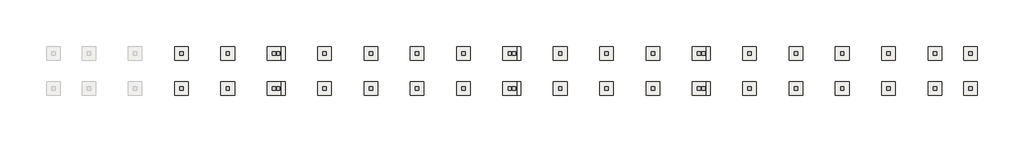
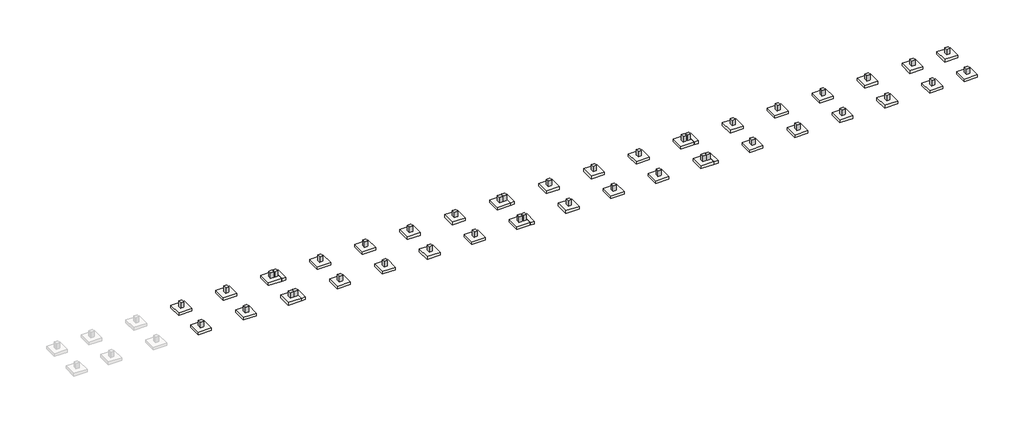
# Not in any storey, part 3 of 3: 42 columns, 42 slabs.
"""IFC4 building model written with IfcOpenShell, lengths in millimetres."""

import ifcopenshell
import ifcopenshell.guid

model = None  # the IFC model being written
_history = None  # IfcOwnerHistory: only IFC2X3 demands one
_inside = {}  # id of a spatial element -> (the spatial element, [elements in it])
_under = {}  # id of a project, library or spatial element -> (it, [spatial elements below it])
_declared = {}  # id of a project -> (the project, [libraries it declares])
_typed = {}  # id of a type object -> (the type object, [elements of that type])
_made_of = {}  # id of a material, layer set ... -> (it, [elements and type objects made of it])


def new_model(schema):
    """Start an empty IFC model of exactly this schema.

    Asked for "IFC4X3", IfcOpenShell would pick the latest addendum, in which some entities
    have other attributes; the version numbers below select the first issue.
    IFC2X3 requires an IfcOwnerHistory on every rooted entity: one is made here for all.
    """
    global model, _history
    if schema == "IFC4X3":
        model = ifcopenshell.file(schema_version=(4, 3, 0, 0))
    else:
        model = ifcopenshell.file(schema=schema)
    _inside.clear()
    _under.clear()
    _declared.clear()
    _typed.clear()
    _made_of.clear()
    _history = None
    if model.schema == "IFC2X3":
        org = make("IfcOrganization", Name="unknown")
        user = make(
            "IfcPersonAndOrganization",
            ThePerson=make("IfcPerson", FamilyName="unknown"),
            TheOrganization=org,
        )
        app = make(
            "IfcApplication",
            ApplicationDeveloper=org,
            Version="unknown",
            ApplicationFullName="unknown",
            ApplicationIdentifier="unknown",
        )
        _history = make(
            "IfcOwnerHistory",
            OwningUser=user,
            OwningApplication=app,
            ChangeAction="ADDED",
            CreationDate=0,
        )
    return model


def make(cls, **values):
    """One entity of the class cls with the attributes given. An attribute that is None is left unset."""
    return model.create_entity(
        cls, **{name: value for name, value in values.items() if value is not None}
    )


def rooted(cls, **values):
    """An entity with a GlobalId (a new one), such as an element, a storey or a relation."""
    return make(cls, GlobalId=ifcopenshell.guid.new(), OwnerHistory=_history, **values)


def si_unit(unit_type, name, prefix=None):
    """IfcSIUnit, for example si_unit("LENGTHUNIT", "METRE", prefix="MILLI")."""
    return make("IfcSIUnit", UnitType=unit_type, Prefix=prefix, Name=name)


def assignment(units):
    """IfcUnitAssignment: the units of a project."""
    return None if units is None else make("IfcUnitAssignment", Units=units)


def point(xyz):
    """IfcCartesianPoint."""
    return None if xyz is None else make("IfcCartesianPoint", Coordinates=xyz)


def direction(xyz):
    """IfcDirection."""
    return None if xyz is None else make("IfcDirection", DirectionRatios=xyz)


def frame(location, z_axis=None, x_axis=None):
    """IfcAxis2Placement3D, a coordinate frame: its origin and axes. An axis left out is left unset."""
    return make(
        "IfcAxis2Placement3D",
        Location=point(location),
        Axis=direction(z_axis),
        RefDirection=direction(x_axis),
    )


def origin():
    """The frame at (0, 0, 0) with its axes left unset."""
    return frame((0.0, 0.0, 0.0))


def place(relative_to, where):
    """IfcLocalPlacement: puts the frame where relative to a parent placement (None: the world)."""
    return make(
        "IfcLocalPlacement", PlacementRelTo=relative_to, RelativePlacement=where
    )


def context(
    kind, dimensions, precision=None, world=None, true_north=None, identifier=None
):
    """IfcGeometricRepresentationContext, for example the 3D "Model" context."""
    return make(
        "IfcGeometricRepresentationContext",
        ContextIdentifier=identifier,
        ContextType=kind,
        CoordinateSpaceDimension=dimensions,
        Precision=precision,
        WorldCoordinateSystem=world,
        TrueNorth=true_north,
    )


def project(units=None, contexts=None):
    """IfcProject with its units and contexts."""
    return rooted(
        "IfcProject",
        Name="project",
        RepresentationContexts=contexts,
        UnitsInContext=assignment(units),
    )


def spatial(cls, under=None, at=None, **own):
    """A site, building, storey or space (cls), placed at a placement, below another one or the project."""
    s = rooted(cls, ObjectPlacement=at, **own)
    if under is not None:
        _under.setdefault(under.id(), (under, []))[1].append(s)
    return s


def polyline(points):
    """IfcPolyline through the points."""
    return make("IfcPolyline", Points=[point(p) for p in points])


def outline(outer, holes=None, kind="AREA"):
    """IfcArbitraryClosedProfileDef: a profile drawn as a closed curve; with holes, ...WithVoids."""
    if holes is None:
        return make("IfcArbitraryClosedProfileDef", ProfileType=kind, OuterCurve=outer)
    return make(
        "IfcArbitraryProfileDefWithVoids",
        ProfileType=kind,
        OuterCurve=outer,
        InnerCurves=holes,
    )


def extrude(swept, where, along, depth):
    """IfcExtrudedAreaSolid: the profile swept, set in the frame where, extruded along a direction by depth."""
    return make(
        "IfcExtrudedAreaSolid",
        SweptArea=swept,
        Position=where,
        ExtrudedDirection=direction(along),
        Depth=depth,
    )


def shape(context_of_items, identifier, shape_type, items):
    """IfcShapeRepresentation: the items that make up one representation, for example the "Body"."""
    return make(
        "IfcShapeRepresentation",
        ContextOfItems=context_of_items,
        RepresentationIdentifier=identifier,
        RepresentationType=shape_type,
        Items=items,
    )


def source(mapping_origin, context_of_items, identifier, shape_type, items):
    """IfcRepresentationMap: a shape defined once, which mapped items show again and again."""
    return make(
        "IfcRepresentationMap",
        MappingOrigin=mapping_origin,
        MappedRepresentation=shape(context_of_items, identifier, shape_type, items),
    )


def transform(
    local_origin,
    x_axis=None,
    y_axis=None,
    z_axis=None,
    scale=None,
    scale2=None,
    scale3=None,
    uniform=True,
):
    """IfcCartesianTransformationOperator3D, or its non-uniform kind. x_axis, y_axis, z_axis: its Axis1, 2, 3."""
    if uniform:
        return make(
            "IfcCartesianTransformationOperator3D",
            Axis1=direction(x_axis),
            Axis2=direction(y_axis),
            LocalOrigin=point(local_origin),
            Scale=scale,
            Axis3=direction(z_axis),
        )
    return make(
        "IfcCartesianTransformationOperator3DnonUniform",
        Axis1=direction(x_axis),
        Axis2=direction(y_axis),
        LocalOrigin=point(local_origin),
        Scale=scale,
        Axis3=direction(z_axis),
        Scale2=scale2,
        Scale3=scale3,
    )


def mapped(mapping_source, mapping_target):
    """IfcMappedItem: shows the shape of a source again, moved by a transform."""
    return make(
        "IfcMappedItem", MappingSource=mapping_source, MappingTarget=mapping_target
    )


def made_of(thing, what):
    """Note that an element or type object is made of a material, layer set ...; save() writes the relation."""
    if what is not None:
        _made_of.setdefault(what.id(), (what, []))[1].append(thing)
    return thing


def element(
    cls,
    number,
    at=None,
    inside=None,
    cuts=None,
    type_object=None,
    material=None,
    context=None,
    identifier="Body",
    shape_type=None,
    held_by="IfcProductDefinitionShape",
    body=None,
    shapes=None,
    **own,
):
    """One element of the class cls, such as IfcWall. Its Tag is "e" and its number.

    at: its placement. inside: the storey or other place that contains it. cuts: it is an
    opening in that element (IfcRelVoidsElement). A single representation is given by context,
    identifier, shape_type and body (its items); several are given by shapes. held_by: the class
    of the entity that holds the representations. save() writes the other relations.
    """
    e = rooted(cls, Tag="e%d" % number, ObjectPlacement=at, **own)
    if body is not None:
        shapes = [shape(context, identifier, shape_type, body)]
    if shapes is not None:
        e.Representation = make(held_by, Representations=shapes)
    if inside is not None:
        _inside.setdefault(inside.id(), (inside, []))[1].append(e)
    if cuts is not None:
        rooted(
            "IfcRelVoidsElement", RelatingBuildingElement=cuts, RelatedOpeningElement=e
        )
    if type_object is not None:
        _typed.setdefault(type_object.id(), (type_object, []))[1].append(e)
    return made_of(e, material)


def aggregate(whole, parts):
    """IfcRelAggregates: a whole, such as a stair, and the parts it consists of."""
    return rooted("IfcRelAggregates", RelatingObject=whole, RelatedObjects=parts)


def save(model, path):
    """Write the relations noted so far, then the file.

    IfcRelAggregates (storeys below a building ...), IfcRelContainedInSpatialStructure (elements
    in a storey), IfcRelDefinesByType, IfcRelAssociatesMaterial and IfcRelDeclares: one each for
    every whole, place, type object, material and project.
    """
    for whole, parts in _under.values():
        aggregate(whole, parts)
    for where, things in _inside.values():
        rooted(
            "IfcRelContainedInSpatialStructure",
            RelatedElements=things,
            RelatingStructure=where,
        )
    for kind, things in _typed.values():
        rooted("IfcRelDefinesByType", RelatedObjects=things, RelatingType=kind)
    for what, things in _made_of.values():
        rooted("IfcRelAssociatesMaterial", RelatedObjects=things, RelatingMaterial=what)
    for by, libraries in _declared.values():
        rooted("IfcRelDeclares", RelatingContext=by, RelatedDefinitions=libraries)
    model.write(path)


def foundation_rectangular_non_pile_5fe39465(model_context):
    return source(origin(), model_context, "Body", "SweptSolid", [
        extrude(outline(polyline([(1200.0, 1200.0), (1200.0, -1200.0), (-1200.0, -1200.0), (-1200.0, 1200.0), (1200.0, 1200.0)])), frame((0.0, 0.0, -500.0), z_axis=(0.0, 0.0, 1.0), x_axis=(1.0, 0.0, 0.0)), (0.0, 0.0, 1.0), 500.0),
    ])


model = new_model("IFC4")

# Units and contexts
model_context = context("Model", 3, world=origin())
ifc_project = project(units=[si_unit("LENGTHUNIT", "METRE", prefix="MILLI")], contexts=[model_context])

# Site, building
site = spatial("IfcSite", under=ifc_project)
building = spatial("IfcBuilding", under=site)

# Columns
placement = place(None, origin())
element("IfcColumn", 1, ObjectType="RC_Column_Rectangular : H_SC_AR_S15_UG PED_W600xL600_Bit_Anchor", at=placement, inside=building, context=model_context, shape_type="SweptSolid", body=[
    extrude(outline(polyline([(18630.0, 549.5208589), (18630.0, -50.4791411), (18030.0, -50.4791411), (18030.0, 549.5208589), (18630.0, 549.5208589)])), frame((0.0, 0.0, -750.0381366), z_axis=(0.0, 0.0, 1.0), x_axis=(1.0, 0.0, 0.0)), (0.0, 0.0, 1.0), 1050.0),
])
element("IfcColumn", 2, ObjectType="RC_Column_Rectangular : H_SC_AR_S15_UG PED_W600xL600_Bit_Anchor", at=placement, inside=building, context=model_context, shape_type="SweptSolid", body=[
    extrude(outline(polyline([(26830.0, 549.5208589), (26830.0, -50.4791411), (26230.0, -50.4791411), (26230.0, 549.5208589), (26830.0, 549.5208589)])), frame((0.0, 0.0, -750.0381366), z_axis=(0.0, 0.0, 1.0), x_axis=(1.0, 0.0, 0.0)), (0.0, 0.0, 1.0), 1050.0),
])
element("IfcColumn", 3, ObjectType="RC_Column_Rectangular : H_SC_AR_S15_UG PED_W600xL600_Bit_Anchor", at=placement, inside=building, context=model_context, shape_type="SweptSolid", body=[
    extrude(outline(polyline([(35030.0, 549.5208589), (35030.0, -50.4791411), (34430.0, -50.4791411), (34430.0, 549.5208589), (35030.0, 549.5208589)])), frame((0.0, 0.0, -750.0381366), z_axis=(0.0, 0.0, 1.0), x_axis=(1.0, 0.0, 0.0)), (0.0, 0.0, 1.0), 1050.0),
])
element("IfcColumn", 4, ObjectType="RC_Column_Rectangular : H_SC_AR_S15_UG PED_W600xL600_Bit_Anchor", at=placement, inside=building, context=model_context, shape_type="SweptSolid", body=[
    extrude(outline(polyline([(35780.0, 549.5208589), (35780.0, -50.4791411), (35180.0, -50.4791411), (35180.0, 549.5208589), (35780.0, 549.5208589)])), frame((0.0, 0.0, -750.0381366), z_axis=(0.0, 0.0, 1.0), x_axis=(1.0, 0.0, 0.0)), (0.0, 0.0, 1.0), 1050.0),
])
element("IfcColumn", 5, ObjectType="RC_Column_Rectangular : H_SC_AR_S15_UG PED_W600xL600_Bit_Anchor", at=placement, inside=building, context=model_context, shape_type="SweptSolid", body=[
    extrude(outline(polyline([(43980.0, 549.5208589), (43980.0, -50.4791411), (43380.0, -50.4791411), (43380.0, 549.5208589), (43980.0, 549.5208589)])), frame((0.0, 0.0, -750.0381366), z_axis=(0.0, 0.0, 1.0), x_axis=(1.0, 0.0, 0.0)), (0.0, 0.0, 1.0), 1050.0),
])
element("IfcColumn", 6, ObjectType="RC_Column_Rectangular : H_SC_AR_S15_UG PED_W600xL600_Bit_Anchor", at=placement, inside=building, context=model_context, shape_type="SweptSolid", body=[
    extrude(outline(polyline([(52180.0, 549.5208589), (52180.0, -50.4791411), (51580.0, -50.4791411), (51580.0, 549.5208589), (52180.0, 549.5208589)])), frame((0.0, 0.0, -750.0381366), z_axis=(0.0, 0.0, 1.0), x_axis=(1.0, 0.0, 0.0)), (0.0, 0.0, 1.0), 1050.0),
])
element("IfcColumn", 7, ObjectType="RC_Column_Rectangular : H_SC_AR_S15_UG PED_W600xL600_Bit_Anchor", at=placement, inside=building, context=model_context, shape_type="SweptSolid", body=[
    extrude(outline(polyline([(60380.0, 549.5208589), (60380.0, -50.4791411), (59780.0, -50.4791411), (59780.0, 549.5208589), (60380.0, 549.5208589)])), frame((0.0, 0.0, -750.0381366), z_axis=(0.0, 0.0, 1.0), x_axis=(1.0, 0.0, 0.0)), (0.0, 0.0, 1.0), 1050.0),
])
element("IfcColumn", 8, ObjectType="RC_Column_Rectangular : H_SC_AR_S15_UG PED_W600xL600_Bit_Anchor", at=placement, inside=building, context=model_context, shape_type="SweptSolid", body=[
    extrude(outline(polyline([(68580.0, 549.5208589), (68580.0, -50.4791411), (67980.0, -50.4791411), (67980.0, 549.5208589), (68580.0, 549.5208589)])), frame((0.0, 0.0, -750.0381366), z_axis=(0.0, 0.0, 1.0), x_axis=(1.0, 0.0, 0.0)), (0.0, 0.0, 1.0), 1050.0),
])
element("IfcColumn", 9, ObjectType="RC_Column_Rectangular : H_SC_AR_S15_UG PED_W600xL600_Bit_Anchor", at=placement, inside=building, context=model_context, shape_type="SweptSolid", body=[
    extrude(outline(polyline([(76780.0, 549.5208589), (76780.0, -50.4791411), (76180.0, -50.4791411), (76180.0, 549.5208589), (76780.0, 549.5208589)])), frame((0.0, 0.0, -750.0381366), z_axis=(0.0, 0.0, 1.0), x_axis=(1.0, 0.0, 0.0)), (0.0, 0.0, 1.0), 1050.0),
])
element("IfcColumn", 10, ObjectType="RC_Column_Rectangular : H_SC_AR_S15_UG PED_W600xL600_Bit_Anchor", at=placement, inside=building, context=model_context, shape_type="SweptSolid", body=[
    extrude(outline(polyline([(77530.0, 549.5208589), (77530.0, -50.4791411), (76930.0, -50.4791411), (76930.0, 549.5208589), (77530.0, 549.5208589)])), frame((0.0, 0.0, -750.0381366), z_axis=(0.0, 0.0, 1.0), x_axis=(1.0, 0.0, 0.0)), (0.0, 0.0, 1.0), 1050.0),
])
element("IfcColumn", 11, ObjectType="RC_Column_Rectangular : H_SC_AR_S15_UG PED_W600xL600_Bit_Anchor", at=placement, inside=building, context=model_context, shape_type="SweptSolid", body=[
    extrude(outline(polyline([(85730.0, 549.5208589), (85730.0, -50.4791411), (85130.0, -50.4791411), (85130.0, 549.5208589), (85730.0, 549.5208589)])), frame((0.0, 0.0, -750.0381366), z_axis=(0.0, 0.0, 1.0), x_axis=(1.0, 0.0, 0.0)), (0.0, 0.0, 1.0), 1050.0),
])
element("IfcColumn", 12, ObjectType="RC_Column_Rectangular : H_SC_AR_S15_UG PED_W600xL600_Bit_Anchor", at=placement, inside=building, context=model_context, shape_type="SweptSolid", body=[
    extrude(outline(polyline([(93930.0, 549.5208589), (93930.0, -50.4791411), (93330.0, -50.4791411), (93330.0, 549.5208589), (93930.0, 549.5208589)])), frame((0.0, 0.0, -750.0381366), z_axis=(0.0, 0.0, 1.0), x_axis=(1.0, 0.0, 0.0)), (0.0, 0.0, 1.0), 1050.0),
])
element("IfcColumn", 13, ObjectType="RC_Column_Rectangular : H_SC_AR_S15_UG PED_W600xL600_Bit_Anchor", at=placement, inside=building, context=model_context, shape_type="SweptSolid", body=[
    extrude(outline(polyline([(102130.0, 549.5208589), (102130.0, -50.4791411), (101530.0, -50.4791411), (101530.0, 549.5208589), (102130.0, 549.5208589)])), frame((0.0, 0.0, -750.0381366), z_axis=(0.0, 0.0, 1.0), x_axis=(1.0, 0.0, 0.0)), (0.0, 0.0, 1.0), 1050.0),
])
element("IfcColumn", 14, ObjectType="RC_Column_Rectangular : H_SC_AR_S15_UG PED_W600xL600_Bit_Anchor", at=placement, inside=building, context=model_context, shape_type="SweptSolid", body=[
    extrude(outline(polyline([(110330.0, 549.5208589), (110330.0, -50.4791411), (109730.0, -50.4791411), (109730.0, 549.5208589), (110330.0, 549.5208589)])), frame((0.0, 0.0, -750.0381366), z_axis=(0.0, 0.0, 1.0), x_axis=(1.0, 0.0, 0.0)), (0.0, 0.0, 1.0), 1050.0),
])
element("IfcColumn", 15, ObjectType="RC_Column_Rectangular : H_SC_AR_S15_UG PED_W600xL600_Bit_Anchor", at=placement, inside=building, context=model_context, shape_type="SweptSolid", body=[
    extrude(outline(polyline([(111080.0, 549.5208589), (111080.0, -50.4791411), (110480.0, -50.4791411), (110480.0, 549.5208589), (111080.0, 549.5208589)])), frame((0.0, 0.0, -750.0381366), z_axis=(0.0, 0.0, 1.0), x_axis=(1.0, 0.0, 0.0)), (0.0, 0.0, 1.0), 1050.0),
])
element("IfcColumn", 16, ObjectType="RC_Column_Rectangular : H_SC_AR_S15_UG PED_W600xL600_Bit_Anchor", at=placement, inside=building, context=model_context, shape_type="SweptSolid", body=[
    extrude(outline(polyline([(119280.0, 549.5208589), (119280.0, -50.4791411), (118680.0, -50.4791411), (118680.0, 549.5208589), (119280.0, 549.5208589)])), frame((0.0, 0.0, -750.0381366), z_axis=(0.0, 0.0, 1.0), x_axis=(1.0, 0.0, 0.0)), (0.0, 0.0, 1.0), 1050.0),
])
element("IfcColumn", 17, ObjectType="RC_Column_Rectangular : H_SC_AR_S15_UG PED_W600xL600_Bit_Anchor", at=placement, inside=building, context=model_context, shape_type="SweptSolid", body=[
    extrude(outline(polyline([(127480.0, 549.5208589), (127480.0, -50.4791411), (126880.0, -50.4791411), (126880.0, 549.5208589), (127480.0, 549.5208589)])), frame((0.0, 0.0, -750.0381366), z_axis=(0.0, 0.0, 1.0), x_axis=(1.0, 0.0, 0.0)), (0.0, 0.0, 1.0), 1050.0),
])
element("IfcColumn", 18, ObjectType="RC_Column_Rectangular : H_SC_AR_S15_UG PED_W600xL600_Bit_Anchor", at=placement, inside=building, context=model_context, shape_type="SweptSolid", body=[
    extrude(outline(polyline([(135680.0, 549.5208589), (135680.0, -50.4791411), (135080.0, -50.4791411), (135080.0, 549.5208589), (135680.0, 549.5208589)])), frame((0.0, 0.0, -750.0381366), z_axis=(0.0, 0.0, 1.0), x_axis=(1.0, 0.0, 0.0)), (0.0, 0.0, 1.0), 1050.0),
])
element("IfcColumn", 19, ObjectType="RC_Column_Rectangular : H_SC_AR_S15_UG PED_W600xL600_Bit_Anchor", at=placement, inside=building, context=model_context, shape_type="SweptSolid", body=[
    extrude(outline(polyline([(143880.0, 549.5208589), (143880.0, -50.4791411), (143280.0, -50.4791411), (143280.0, 549.5208589), (143880.0, 549.5208589)])), frame((0.0, 0.0, -750.0381366), z_axis=(0.0, 0.0, 1.0), x_axis=(1.0, 0.0, 0.0)), (0.0, 0.0, 1.0), 1050.0),
])
element("IfcColumn", 20, ObjectType="RC_Column_Rectangular : H_SC_AR_S15_UG PED_W600xL600_Bit_Anchor", at=placement, inside=building, context=model_context, shape_type="SweptSolid", body=[
    extrude(outline(polyline([(152080.0, 549.5208589), (152080.0, -50.4791411), (151480.0, -50.4791411), (151480.0, 549.5208589), (152080.0, 549.5208589)])), frame((0.0, 0.0, -750.0381366), z_axis=(0.0, 0.0, 1.0), x_axis=(1.0, 0.0, 0.0)), (0.0, 0.0, 1.0), 1050.0),
])
element("IfcColumn", 21, ObjectType="RC_Column_Rectangular : H_SC_AR_S15_UG PED_W600xL600_Bit_Anchor", at=placement, inside=building, context=model_context, shape_type="SweptSolid", body=[
    extrude(outline(polyline([(158430.0, 549.5208589), (158430.0, -50.4791411), (157830.0, -50.4791411), (157830.0, 549.5208589), (158430.0, 549.5208589)])), frame((0.0, 0.0, -750.0381366), z_axis=(0.0, 0.0, 1.0), x_axis=(1.0, 0.0, 0.0)), (0.0, 0.0, 1.0), 1050.0),
])
element("IfcColumn", 22, ObjectType="RC_Column_Rectangular : H_SC_AR_S15_UG PED_W600xL600_Bit_Anchor", at=placement, inside=building, context=model_context, shape_type="SweptSolid", body=[
    extrude(outline(polyline([(18630.0, 6799.5208589), (18630.0, 6199.5208589), (18030.0, 6199.5208589), (18030.0, 6799.5208589), (18630.0, 6799.5208589)])), frame((0.0, 0.0, -750.0381366), z_axis=(0.0, 0.0, 1.0), x_axis=(1.0, 0.0, 0.0)), (0.0, 0.0, 1.0), 1050.0),
])
element("IfcColumn", 23, ObjectType="RC_Column_Rectangular : H_SC_AR_S15_UG PED_W600xL600_Bit_Anchor", at=placement, inside=building, context=model_context, shape_type="SweptSolid", body=[
    extrude(outline(polyline([(26830.0, 6799.5208589), (26830.0, 6199.5208589), (26230.0, 6199.5208589), (26230.0, 6799.5208589), (26830.0, 6799.5208589)])), frame((0.0, 0.0, -750.0381366), z_axis=(0.0, 0.0, 1.0), x_axis=(1.0, 0.0, 0.0)), (0.0, 0.0, 1.0), 1050.0),
])
element("IfcColumn", 24, ObjectType="RC_Column_Rectangular : H_SC_AR_S15_UG PED_W600xL600_Bit_Anchor", at=placement, inside=building, context=model_context, shape_type="SweptSolid", body=[
    extrude(outline(polyline([(35030.0, 6799.5208589), (35030.0, 6199.5208589), (34430.0, 6199.5208589), (34430.0, 6799.5208589), (35030.0, 6799.5208589)])), frame((0.0, 0.0, -750.0381366), z_axis=(0.0, 0.0, 1.0), x_axis=(1.0, 0.0, 0.0)), (0.0, 0.0, 1.0), 1050.0),
])
element("IfcColumn", 25, ObjectType="RC_Column_Rectangular : H_SC_AR_S15_UG PED_W600xL600_Bit_Anchor", at=placement, inside=building, context=model_context, shape_type="SweptSolid", body=[
    extrude(outline(polyline([(35780.0, 6799.5208589), (35780.0, 6199.5208589), (35180.0, 6199.5208589), (35180.0, 6799.5208589), (35780.0, 6799.5208589)])), frame((0.0, 0.0, -750.0381366), z_axis=(0.0, 0.0, 1.0), x_axis=(1.0, 0.0, 0.0)), (0.0, 0.0, 1.0), 1050.0),
])
element("IfcColumn", 26, ObjectType="RC_Column_Rectangular : H_SC_AR_S15_UG PED_W600xL600_Bit_Anchor", at=placement, inside=building, context=model_context, shape_type="SweptSolid", body=[
    extrude(outline(polyline([(43980.0, 6799.5208589), (43980.0, 6199.5208589), (43380.0, 6199.5208589), (43380.0, 6799.5208589), (43980.0, 6799.5208589)])), frame((0.0, 0.0, -750.0381366), z_axis=(0.0, 0.0, 1.0), x_axis=(1.0, 0.0, 0.0)), (0.0, 0.0, 1.0), 1050.0),
])
element("IfcColumn", 27, ObjectType="RC_Column_Rectangular : H_SC_AR_S15_UG PED_W600xL600_Bit_Anchor", at=placement, inside=building, context=model_context, shape_type="SweptSolid", body=[
    extrude(outline(polyline([(52180.0, 6799.5208589), (52180.0, 6199.5208589), (51580.0, 6199.5208589), (51580.0, 6799.5208589), (52180.0, 6799.5208589)])), frame((0.0, 0.0, -750.0381366), z_axis=(0.0, 0.0, 1.0), x_axis=(1.0, 0.0, 0.0)), (0.0, 0.0, 1.0), 1050.0),
])
element("IfcColumn", 28, ObjectType="RC_Column_Rectangular : H_SC_AR_S15_UG PED_W600xL600_Bit_Anchor", at=placement, inside=building, context=model_context, shape_type="SweptSolid", body=[
    extrude(outline(polyline([(60380.0, 6799.5208589), (60380.0, 6199.5208589), (59780.0, 6199.5208589), (59780.0, 6799.5208589), (60380.0, 6799.5208589)])), frame((0.0, 0.0, -750.0381366), z_axis=(0.0, 0.0, 1.0), x_axis=(1.0, 0.0, 0.0)), (0.0, 0.0, 1.0), 1050.0),
])
element("IfcColumn", 29, ObjectType="RC_Column_Rectangular : H_SC_AR_S15_UG PED_W600xL600_Bit_Anchor", at=placement, inside=building, context=model_context, shape_type="SweptSolid", body=[
    extrude(outline(polyline([(68580.0, 6799.5208589), (68580.0, 6199.5208589), (67980.0, 6199.5208589), (67980.0, 6799.5208589), (68580.0, 6799.5208589)])), frame((0.0, 0.0, -750.0381366), z_axis=(0.0, 0.0, 1.0), x_axis=(1.0, 0.0, 0.0)), (0.0, 0.0, 1.0), 1050.0),
])
element("IfcColumn", 30, ObjectType="RC_Column_Rectangular : H_SC_AR_S15_UG PED_W600xL600_Bit_Anchor", at=placement, inside=building, context=model_context, shape_type="SweptSolid", body=[
    extrude(outline(polyline([(76780.0, 6799.5208589), (76780.0, 6199.5208589), (76180.0, 6199.5208589), (76180.0, 6799.5208589), (76780.0, 6799.5208589)])), frame((0.0, 0.0, -750.0381366), z_axis=(0.0, 0.0, 1.0), x_axis=(1.0, 0.0, 0.0)), (0.0, 0.0, 1.0), 1050.0),
])
element("IfcColumn", 31, ObjectType="RC_Column_Rectangular : H_SC_AR_S15_UG PED_W600xL600_Bit_Anchor", at=placement, inside=building, context=model_context, shape_type="SweptSolid", body=[
    extrude(outline(polyline([(77530.0, 6799.5208589), (77530.0, 6199.5208589), (76930.0, 6199.5208589), (76930.0, 6799.5208589), (77530.0, 6799.5208589)])), frame((0.0, 0.0, -750.0381366), z_axis=(0.0, 0.0, 1.0), x_axis=(1.0, 0.0, 0.0)), (0.0, 0.0, 1.0), 1050.0),
])
element("IfcColumn", 32, ObjectType="RC_Column_Rectangular : H_SC_AR_S15_UG PED_W600xL600_Bit_Anchor", at=placement, inside=building, context=model_context, shape_type="SweptSolid", body=[
    extrude(outline(polyline([(85730.0, 6799.5208589), (85730.0, 6199.5208589), (85130.0, 6199.5208589), (85130.0, 6799.5208589), (85730.0, 6799.5208589)])), frame((0.0, 0.0, -750.0381366), z_axis=(0.0, 0.0, 1.0), x_axis=(1.0, 0.0, 0.0)), (0.0, 0.0, 1.0), 1050.0),
])
element("IfcColumn", 33, ObjectType="RC_Column_Rectangular : H_SC_AR_S15_UG PED_W600xL600_Bit_Anchor", at=placement, inside=building, context=model_context, shape_type="SweptSolid", body=[
    extrude(outline(polyline([(93930.0, 6799.5208589), (93930.0, 6199.5208589), (93330.0, 6199.5208589), (93330.0, 6799.5208589), (93930.0, 6799.5208589)])), frame((0.0, 0.0, -750.0381366), z_axis=(0.0, 0.0, 1.0), x_axis=(1.0, 0.0, 0.0)), (0.0, 0.0, 1.0), 1050.0),
])
element("IfcColumn", 34, ObjectType="RC_Column_Rectangular : H_SC_AR_S15_UG PED_W600xL600_Bit_Anchor", at=placement, inside=building, context=model_context, shape_type="SweptSolid", body=[
    extrude(outline(polyline([(102130.0, 6799.5208589), (102130.0, 6199.5208589), (101530.0, 6199.5208589), (101530.0, 6799.5208589), (102130.0, 6799.5208589)])), frame((0.0, 0.0, -750.0381366), z_axis=(0.0, 0.0, 1.0), x_axis=(1.0, 0.0, 0.0)), (0.0, 0.0, 1.0), 1050.0),
])
element("IfcColumn", 35, ObjectType="RC_Column_Rectangular : H_SC_AR_S15_UG PED_W600xL600_Bit_Anchor", at=placement, inside=building, context=model_context, shape_type="SweptSolid", body=[
    extrude(outline(polyline([(110330.0, 6799.5208589), (110330.0, 6199.5208589), (109730.0, 6199.5208589), (109730.0, 6799.5208589), (110330.0, 6799.5208589)])), frame((0.0, 0.0, -750.0381366), z_axis=(0.0, 0.0, 1.0), x_axis=(1.0, 0.0, 0.0)), (0.0, 0.0, 1.0), 1050.0),
])
element("IfcColumn", 36, ObjectType="RC_Column_Rectangular : H_SC_AR_S15_UG PED_W600xL600_Bit_Anchor", at=placement, inside=building, context=model_context, shape_type="SweptSolid", body=[
    extrude(outline(polyline([(111080.0, 6799.5208589), (111080.0, 6199.5208589), (110480.0, 6199.5208589), (110480.0, 6799.5208589), (111080.0, 6799.5208589)])), frame((0.0, 0.0, -750.0381366), z_axis=(0.0, 0.0, 1.0), x_axis=(1.0, 0.0, 0.0)), (0.0, 0.0, 1.0), 1050.0),
])
element("IfcColumn", 37, ObjectType="RC_Column_Rectangular : H_SC_AR_S15_UG PED_W600xL600_Bit_Anchor", at=placement, inside=building, context=model_context, shape_type="SweptSolid", body=[
    extrude(outline(polyline([(119280.0, 6799.5208589), (119280.0, 6199.5208589), (118680.0, 6199.5208589), (118680.0, 6799.5208589), (119280.0, 6799.5208589)])), frame((0.0, 0.0, -750.0381366), z_axis=(0.0, 0.0, 1.0), x_axis=(1.0, 0.0, 0.0)), (0.0, 0.0, 1.0), 1050.0),
])
element("IfcColumn", 38, ObjectType="RC_Column_Rectangular : H_SC_AR_S15_UG PED_W600xL600_Bit_Anchor", at=placement, inside=building, context=model_context, shape_type="SweptSolid", body=[
    extrude(outline(polyline([(127480.0, 6799.5208589), (127480.0, 6199.5208589), (126880.0, 6199.5208589), (126880.0, 6799.5208589), (127480.0, 6799.5208589)])), frame((0.0, 0.0, -750.0381366), z_axis=(0.0, 0.0, 1.0), x_axis=(1.0, 0.0, 0.0)), (0.0, 0.0, 1.0), 1050.0),
])
element("IfcColumn", 39, ObjectType="RC_Column_Rectangular : H_SC_AR_S15_UG PED_W600xL600_Bit_Anchor", at=placement, inside=building, context=model_context, shape_type="SweptSolid", body=[
    extrude(outline(polyline([(135680.0, 6799.5208589), (135680.0, 6199.5208589), (135080.0, 6199.5208589), (135080.0, 6799.5208589), (135680.0, 6799.5208589)])), frame((0.0, 0.0, -750.0381366), z_axis=(0.0, 0.0, 1.0), x_axis=(1.0, 0.0, 0.0)), (0.0, 0.0, 1.0), 1050.0),
])
element("IfcColumn", 40, ObjectType="RC_Column_Rectangular : H_SC_AR_S15_UG PED_W600xL600_Bit_Anchor", at=placement, inside=building, context=model_context, shape_type="SweptSolid", body=[
    extrude(outline(polyline([(143880.0, 6799.5208589), (143880.0, 6199.5208589), (143280.0, 6199.5208589), (143280.0, 6799.5208589), (143880.0, 6799.5208589)])), frame((0.0, 0.0, -750.0381366), z_axis=(0.0, 0.0, 1.0), x_axis=(1.0, 0.0, 0.0)), (0.0, 0.0, 1.0), 1050.0),
])
element("IfcColumn", 41, ObjectType="RC_Column_Rectangular : H_SC_AR_S15_UG PED_W600xL600_Bit_Anchor", at=placement, inside=building, context=model_context, shape_type="SweptSolid", body=[
    extrude(outline(polyline([(152080.0, 6799.5208589), (152080.0, 6199.5208589), (151480.0, 6199.5208589), (151480.0, 6799.5208589), (152080.0, 6799.5208589)])), frame((0.0, 0.0, -750.0381366), z_axis=(0.0, 0.0, 1.0), x_axis=(1.0, 0.0, 0.0)), (0.0, 0.0, 1.0), 1050.0),
])
element("IfcColumn", 42, ObjectType="RC_Column_Rectangular : H_SC_AR_S15_UG PED_W600xL600_Bit_Anchor", at=placement, inside=building, context=model_context, shape_type="SweptSolid", body=[
    extrude(outline(polyline([(158430.0, 6799.5208589), (158430.0, 6199.5208589), (157830.0, 6199.5208589), (157830.0, 6799.5208589), (158430.0, 6799.5208589)])), frame((0.0, 0.0, -750.0381366), z_axis=(0.0, 0.0, 1.0), x_axis=(1.0, 0.0, 0.0)), (0.0, 0.0, 1.0), 1050.0),
])

# Slabs
element("IfcSlab", 43, ObjectType="Foundation Rectangular (Non-Pile) : H_SF_AR_S18_W2400xL2400xT500_Bitumen", at=placement, inside=building, context=model_context, shape_type="SweptSolid", body=[
    extrude(outline(polyline([(35930.0, 1449.5208589), (35930.0, -950.4791411), (33530.0, -950.4791411), (33530.0, 1449.5208589), (35930.0, 1449.5208589)])), frame((0.0, 0.0, -1250.0381366), z_axis=(0.0, 0.0, 1.0), x_axis=(1.0, 0.0, 0.0)), (0.0, 0.0, 1.0), 500.0),
])
element("IfcSlab", 44, ObjectType="Foundation Rectangular (Non-Pile) : H_SF_AR_S18_W2400xL2400xT500_Bitumen", at=placement, inside=building, context=model_context, shape_type="SweptSolid", body=[
    extrude(outline(polyline([(36680.0, 1449.5208589), (36680.0, -950.4791411), (35930.0, -950.4791411), (35930.0, 1449.5208589), (36680.0, 1449.5208589)])), frame((0.0, 0.0, -1250.0381366), z_axis=(0.0, 0.0, 1.0), x_axis=(1.0, 0.0, 0.0)), (0.0, 0.0, 1.0), 500.0),
])
element("IfcSlab", 45, ObjectType="Foundation Rectangular (Non-Pile) : H_SF_AR_S18_W2400xL2400xT500_Bitumen", at=placement, inside=building, context=model_context, shape_type="SweptSolid", body=[
    extrude(outline(polyline([(77680.0, 1449.5208589), (77680.0, -950.4791411), (75280.0, -950.4791411), (75280.0, 1449.5208589), (77680.0, 1449.5208589)])), frame((0.0, 0.0, -1250.0381366), z_axis=(0.0, 0.0, 1.0), x_axis=(1.0, 0.0, 0.0)), (0.0, 0.0, 1.0), 500.0),
])
element("IfcSlab", 46, ObjectType="Foundation Rectangular (Non-Pile) : H_SF_AR_S18_W2400xL2400xT500_Bitumen", at=placement, inside=building, context=model_context, shape_type="SweptSolid", body=[
    extrude(outline(polyline([(78430.0, 1449.5208589), (78430.0, -950.4791411), (77680.0, -950.4791411), (77680.0, 1449.5208589), (78430.0, 1449.5208589)])), frame((0.0, 0.0, -1250.0381366), z_axis=(0.0, 0.0, 1.0), x_axis=(1.0, 0.0, 0.0)), (0.0, 0.0, 1.0), 500.0),
])
element("IfcSlab", 47, ObjectType="Foundation Rectangular (Non-Pile) : H_SF_AR_S18_W2400xL2400xT500_Bitumen", at=placement, inside=building, context=model_context, shape_type="SweptSolid", body=[
    extrude(outline(polyline([(111230.0, 1449.5208589), (111230.0, -950.4791411), (108830.0, -950.4791411), (108830.0, 1449.5208589), (111230.0, 1449.5208589)])), frame((0.0, 0.0, -1250.0381366), z_axis=(0.0, 0.0, 1.0), x_axis=(1.0, 0.0, 0.0)), (0.0, 0.0, 1.0), 500.0),
])
element("IfcSlab", 48, ObjectType="Foundation Rectangular (Non-Pile) : H_SF_AR_S18_W2400xL2400xT500_Bitumen", at=placement, inside=building, context=model_context, shape_type="SweptSolid", body=[
    extrude(outline(polyline([(111980.0, 1449.5208589), (111980.0, -950.4791411), (111230.0, -950.4791411), (111230.0, 1449.5208589), (111980.0, 1449.5208589)])), frame((0.0, 0.0, -1250.0381366), z_axis=(0.0, 0.0, 1.0), x_axis=(1.0, 0.0, 0.0)), (0.0, 0.0, 1.0), 500.0),
])
element("IfcSlab", 49, ObjectType="Foundation Rectangular (Non-Pile) : H_SF_AR_S18_W2400xL2400xT500_Bitumen", at=placement, inside=building, context=model_context, shape_type="SweptSolid", body=[
    extrude(outline(polyline([(35930.0, 7699.5208589), (35930.0, 5299.5208589), (33530.0, 5299.5208589), (33530.0, 7699.5208589), (35930.0, 7699.5208589)])), frame((0.0, 0.0, -1250.0381366), z_axis=(0.0, 0.0, 1.0), x_axis=(1.0, 0.0, 0.0)), (0.0, 0.0, 1.0), 500.0),
])
element("IfcSlab", 50, ObjectType="Foundation Rectangular (Non-Pile) : H_SF_AR_S18_W2400xL2400xT500_Bitumen", at=placement, inside=building, context=model_context, shape_type="SweptSolid", body=[
    extrude(outline(polyline([(36680.0, 7699.5208589), (36680.0, 5299.5208589), (35930.0, 5299.5208589), (35930.0, 7699.5208589), (36680.0, 7699.5208589)])), frame((0.0, 0.0, -1250.0381366), z_axis=(0.0, 0.0, 1.0), x_axis=(1.0, 0.0, 0.0)), (0.0, 0.0, 1.0), 500.0),
])
element("IfcSlab", 51, ObjectType="Foundation Rectangular (Non-Pile) : H_SF_AR_S18_W2400xL2400xT500_Bitumen", at=placement, inside=building, context=model_context, shape_type="SweptSolid", body=[
    extrude(outline(polyline([(77680.0, 7699.5208589), (77680.0, 5299.5208589), (75280.0, 5299.5208589), (75280.0, 7699.5208589), (77680.0, 7699.5208589)])), frame((0.0, 0.0, -1250.0381366), z_axis=(0.0, 0.0, 1.0), x_axis=(1.0, 0.0, 0.0)), (0.0, 0.0, 1.0), 500.0),
])
element("IfcSlab", 52, ObjectType="Foundation Rectangular (Non-Pile) : H_SF_AR_S18_W2400xL2400xT500_Bitumen", at=placement, inside=building, context=model_context, shape_type="SweptSolid", body=[
    extrude(outline(polyline([(78430.0, 7699.5208589), (78430.0, 5299.5208589), (77680.0, 5299.5208589), (77680.0, 7699.5208589), (78430.0, 7699.5208589)])), frame((0.0, 0.0, -1250.0381366), z_axis=(0.0, 0.0, 1.0), x_axis=(1.0, 0.0, 0.0)), (0.0, 0.0, 1.0), 500.0),
])
element("IfcSlab", 53, ObjectType="Foundation Rectangular (Non-Pile) : H_SF_AR_S18_W2400xL2400xT500_Bitumen", at=placement, inside=building, context=model_context, shape_type="SweptSolid", body=[
    extrude(outline(polyline([(111230.0, 7699.5208589), (111230.0, 5299.5208589), (108830.0, 5299.5208589), (108830.0, 7699.5208589), (111230.0, 7699.5208589)])), frame((0.0, 0.0, -1250.0381366), z_axis=(0.0, 0.0, 1.0), x_axis=(1.0, 0.0, 0.0)), (0.0, 0.0, 1.0), 500.0),
])
element("IfcSlab", 54, ObjectType="Foundation Rectangular (Non-Pile) : H_SF_AR_S18_W2400xL2400xT500_Bitumen", at=placement, inside=building, context=model_context, shape_type="SweptSolid", body=[
    extrude(outline(polyline([(111980.0, 7699.5208589), (111980.0, 5299.5208589), (111230.0, 5299.5208589), (111230.0, 7699.5208589), (111980.0, 7699.5208589)])), frame((0.0, 0.0, -1250.0381366), z_axis=(0.0, 0.0, 1.0), x_axis=(1.0, 0.0, 0.0)), (0.0, 0.0, 1.0), 500.0),
])
foundation_rectangular_non_pile_shape = foundation_rectangular_non_pile_5fe39465(model_context)
element("IfcSlab", 55, ObjectType="Foundation Rectangular (Non-Pile) : H_SF_AR_S18_W2400xL2400xT500_Bitumen", at=placement, inside=building, context=model_context, shape_type="MappedRepresentation", body=[
    mapped(foundation_rectangular_non_pile_shape, transform((18330.0, 249.5208589, -750.0381366), x_axis=(1.0, 0.0, 0.0), y_axis=(0.0, 1.0, 0.0), z_axis=(0.0, 0.0, 1.0))),
])
element("IfcSlab", 56, ObjectType="Foundation Rectangular (Non-Pile) : H_SF_AR_S18_W2400xL2400xT500_Bitumen", at=placement, inside=building, context=model_context, shape_type="MappedRepresentation", body=[
    mapped(foundation_rectangular_non_pile_shape, transform((26530.0, 249.5208589, -750.0381366), x_axis=(1.0, 0.0, 0.0), y_axis=(0.0, 1.0, 0.0), z_axis=(0.0, 0.0, 1.0))),
])
element("IfcSlab", 57, ObjectType="Foundation Rectangular (Non-Pile) : H_SF_AR_S18_W2400xL2400xT500_Bitumen", at=placement, inside=building, context=model_context, shape_type="MappedRepresentation", body=[
    mapped(foundation_rectangular_non_pile_shape, transform((43680.0, 249.5208589, -750.0381366), x_axis=(1.0, 0.0, 0.0), y_axis=(0.0, 1.0, 0.0), z_axis=(0.0, 0.0, 1.0))),
])
element("IfcSlab", 58, ObjectType="Foundation Rectangular (Non-Pile) : H_SF_AR_S18_W2400xL2400xT500_Bitumen", at=placement, inside=building, context=model_context, shape_type="MappedRepresentation", body=[
    mapped(foundation_rectangular_non_pile_shape, transform((51880.0, 249.5208589, -750.0381366), x_axis=(1.0, 0.0, 0.0), y_axis=(0.0, 1.0, 0.0), z_axis=(0.0, 0.0, 1.0))),
])
element("IfcSlab", 59, ObjectType="Foundation Rectangular (Non-Pile) : H_SF_AR_S18_W2400xL2400xT500_Bitumen", at=placement, inside=building, context=model_context, shape_type="MappedRepresentation", body=[
    mapped(foundation_rectangular_non_pile_shape, transform((60080.0, 249.5208589, -750.0381366), x_axis=(1.0, 0.0, 0.0), y_axis=(0.0, 1.0, 0.0), z_axis=(0.0, 0.0, 1.0))),
])
element("IfcSlab", 60, ObjectType="Foundation Rectangular (Non-Pile) : H_SF_AR_S18_W2400xL2400xT500_Bitumen", at=placement, inside=building, context=model_context, shape_type="MappedRepresentation", body=[
    mapped(foundation_rectangular_non_pile_shape, transform((68280.0, 249.5208589, -750.0381366), x_axis=(1.0, 0.0, 0.0), y_axis=(0.0, 1.0, 0.0), z_axis=(0.0, 0.0, 1.0))),
])
element("IfcSlab", 61, ObjectType="Foundation Rectangular (Non-Pile) : H_SF_AR_S18_W2400xL2400xT500_Bitumen", at=placement, inside=building, context=model_context, shape_type="MappedRepresentation", body=[
    mapped(foundation_rectangular_non_pile_shape, transform((85430.0, 249.5208589, -750.0381366), x_axis=(1.0, 0.0, 0.0), y_axis=(0.0, 1.0, 0.0), z_axis=(0.0, 0.0, 1.0))),
])
element("IfcSlab", 62, ObjectType="Foundation Rectangular (Non-Pile) : H_SF_AR_S18_W2400xL2400xT500_Bitumen", at=placement, inside=building, context=model_context, shape_type="MappedRepresentation", body=[
    mapped(foundation_rectangular_non_pile_shape, transform((93630.0, 249.5208589, -750.0381366), x_axis=(1.0, 0.0, 0.0), y_axis=(0.0, 1.0, 0.0), z_axis=(0.0, 0.0, 1.0))),
])
element("IfcSlab", 63, ObjectType="Foundation Rectangular (Non-Pile) : H_SF_AR_S18_W2400xL2400xT500_Bitumen", at=placement, inside=building, context=model_context, shape_type="MappedRepresentation", body=[
    mapped(foundation_rectangular_non_pile_shape, transform((101830.0, 249.5208589, -750.0381366), x_axis=(1.0, 0.0, 0.0), y_axis=(0.0, 1.0, 0.0), z_axis=(0.0, 0.0, 1.0))),
])
element("IfcSlab", 64, ObjectType="Foundation Rectangular (Non-Pile) : H_SF_AR_S18_W2400xL2400xT500_Bitumen", at=placement, inside=building, context=model_context, shape_type="MappedRepresentation", body=[
    mapped(foundation_rectangular_non_pile_shape, transform((118980.0, 249.5208589, -750.0381366), x_axis=(1.0, 0.0, 0.0), y_axis=(0.0, 1.0, 0.0), z_axis=(0.0, 0.0, 1.0))),
])
element("IfcSlab", 65, ObjectType="Foundation Rectangular (Non-Pile) : H_SF_AR_S18_W2400xL2400xT500_Bitumen", at=placement, inside=building, context=model_context, shape_type="MappedRepresentation", body=[
    mapped(foundation_rectangular_non_pile_shape, transform((127180.0, 249.5208589, -750.0381366), x_axis=(1.0, 0.0, 0.0), y_axis=(0.0, 1.0, 0.0), z_axis=(0.0, 0.0, 1.0))),
])
element("IfcSlab", 66, ObjectType="Foundation Rectangular (Non-Pile) : H_SF_AR_S18_W2400xL2400xT500_Bitumen", at=placement, inside=building, context=model_context, shape_type="MappedRepresentation", body=[
    mapped(foundation_rectangular_non_pile_shape, transform((135380.0, 249.5208589, -750.0381366), x_axis=(1.0, 0.0, 0.0), y_axis=(0.0, 1.0, 0.0), z_axis=(0.0, 0.0, 1.0))),
])
element("IfcSlab", 67, ObjectType="Foundation Rectangular (Non-Pile) : H_SF_AR_S18_W2400xL2400xT500_Bitumen", at=placement, inside=building, context=model_context, shape_type="MappedRepresentation", body=[
    mapped(foundation_rectangular_non_pile_shape, transform((143580.0, 249.5208589, -750.0381366), x_axis=(1.0, 0.0, 0.0), y_axis=(0.0, 1.0, 0.0), z_axis=(0.0, 0.0, 1.0))),
])
element("IfcSlab", 68, ObjectType="Foundation Rectangular (Non-Pile) : H_SF_AR_S18_W2400xL2400xT500_Bitumen", at=placement, inside=building, context=model_context, shape_type="MappedRepresentation", body=[
    mapped(foundation_rectangular_non_pile_shape, transform((151780.0, 249.5208589, -750.0381366), x_axis=(1.0, 0.0, 0.0), y_axis=(0.0, 1.0, 0.0), z_axis=(0.0, 0.0, 1.0))),
])
element("IfcSlab", 69, ObjectType="Foundation Rectangular (Non-Pile) : H_SF_AR_S18_W2400xL2400xT500_Bitumen", at=placement, inside=building, context=model_context, shape_type="MappedRepresentation", body=[
    mapped(foundation_rectangular_non_pile_shape, transform((158130.0, 249.5208589, -750.0381366), x_axis=(1.0, 0.0, 0.0), y_axis=(0.0, 1.0, 0.0), z_axis=(0.0, 0.0, 1.0))),
])
element("IfcSlab", 70, ObjectType="Foundation Rectangular (Non-Pile) : H_SF_AR_S18_W2400xL2400xT500_Bitumen", at=placement, inside=building, context=model_context, shape_type="MappedRepresentation", body=[
    mapped(foundation_rectangular_non_pile_shape, transform((18330.0, 6499.5208589, -750.0381366), x_axis=(1.0, 0.0, 0.0), y_axis=(0.0, 1.0, 0.0), z_axis=(0.0, 0.0, 1.0))),
])
element("IfcSlab", 71, ObjectType="Foundation Rectangular (Non-Pile) : H_SF_AR_S18_W2400xL2400xT500_Bitumen", at=placement, inside=building, context=model_context, shape_type="MappedRepresentation", body=[
    mapped(foundation_rectangular_non_pile_shape, transform((26530.0, 6499.5208589, -750.0381366), x_axis=(1.0, 0.0, 0.0), y_axis=(0.0, 1.0, 0.0), z_axis=(0.0, 0.0, 1.0))),
])
element("IfcSlab", 72, ObjectType="Foundation Rectangular (Non-Pile) : H_SF_AR_S18_W2400xL2400xT500_Bitumen", at=placement, inside=building, context=model_context, shape_type="MappedRepresentation", body=[
    mapped(foundation_rectangular_non_pile_shape, transform((43680.0, 6499.5208589, -750.0381366), x_axis=(1.0, 0.0, 0.0), y_axis=(0.0, 1.0, 0.0), z_axis=(0.0, 0.0, 1.0))),
])
element("IfcSlab", 73, ObjectType="Foundation Rectangular (Non-Pile) : H_SF_AR_S18_W2400xL2400xT500_Bitumen", at=placement, inside=building, context=model_context, shape_type="MappedRepresentation", body=[
    mapped(foundation_rectangular_non_pile_shape, transform((51880.0, 6499.5208589, -750.0381366), x_axis=(1.0, 0.0, 0.0), y_axis=(0.0, 1.0, 0.0), z_axis=(0.0, 0.0, 1.0))),
])
element("IfcSlab", 74, ObjectType="Foundation Rectangular (Non-Pile) : H_SF_AR_S18_W2400xL2400xT500_Bitumen", at=placement, inside=building, context=model_context, shape_type="MappedRepresentation", body=[
    mapped(foundation_rectangular_non_pile_shape, transform((60080.0, 6499.5208589, -750.0381366), x_axis=(1.0, 0.0, 0.0), y_axis=(0.0, 1.0, 0.0), z_axis=(0.0, 0.0, 1.0))),
])
element("IfcSlab", 75, ObjectType="Foundation Rectangular (Non-Pile) : H_SF_AR_S18_W2400xL2400xT500_Bitumen", at=placement, inside=building, context=model_context, shape_type="MappedRepresentation", body=[
    mapped(foundation_rectangular_non_pile_shape, transform((68280.0, 6499.5208589, -750.0381366), x_axis=(1.0, 0.0, 0.0), y_axis=(0.0, 1.0, 0.0), z_axis=(0.0, 0.0, 1.0))),
])
element("IfcSlab", 76, ObjectType="Foundation Rectangular (Non-Pile) : H_SF_AR_S18_W2400xL2400xT500_Bitumen", at=placement, inside=building, context=model_context, shape_type="MappedRepresentation", body=[
    mapped(foundation_rectangular_non_pile_shape, transform((85430.0, 6499.5208589, -750.0381366), x_axis=(1.0, 0.0, 0.0), y_axis=(0.0, 1.0, 0.0), z_axis=(0.0, 0.0, 1.0))),
])
element("IfcSlab", 77, ObjectType="Foundation Rectangular (Non-Pile) : H_SF_AR_S18_W2400xL2400xT500_Bitumen", at=placement, inside=building, context=model_context, shape_type="MappedRepresentation", body=[
    mapped(foundation_rectangular_non_pile_shape, transform((93630.0, 6499.5208589, -750.0381366), x_axis=(1.0, 0.0, 0.0), y_axis=(0.0, 1.0, 0.0), z_axis=(0.0, 0.0, 1.0))),
])
element("IfcSlab", 78, ObjectType="Foundation Rectangular (Non-Pile) : H_SF_AR_S18_W2400xL2400xT500_Bitumen", at=placement, inside=building, context=model_context, shape_type="MappedRepresentation", body=[
    mapped(foundation_rectangular_non_pile_shape, transform((101830.0, 6499.5208589, -750.0381366), x_axis=(1.0, 0.0, 0.0), y_axis=(0.0, 1.0, 0.0), z_axis=(0.0, 0.0, 1.0))),
])
element("IfcSlab", 79, ObjectType="Foundation Rectangular (Non-Pile) : H_SF_AR_S18_W2400xL2400xT500_Bitumen", at=placement, inside=building, context=model_context, shape_type="MappedRepresentation", body=[
    mapped(foundation_rectangular_non_pile_shape, transform((118980.0, 6499.5208589, -750.0381366), x_axis=(1.0, 0.0, 0.0), y_axis=(0.0, 1.0, 0.0), z_axis=(0.0, 0.0, 1.0))),
])
element("IfcSlab", 80, ObjectType="Foundation Rectangular (Non-Pile) : H_SF_AR_S18_W2400xL2400xT500_Bitumen", at=placement, inside=building, context=model_context, shape_type="MappedRepresentation", body=[
    mapped(foundation_rectangular_non_pile_shape, transform((127180.0, 6499.5208589, -750.0381366), x_axis=(1.0, 0.0, 0.0), y_axis=(0.0, 1.0, 0.0), z_axis=(0.0, 0.0, 1.0))),
])
element("IfcSlab", 81, ObjectType="Foundation Rectangular (Non-Pile) : H_SF_AR_S18_W2400xL2400xT500_Bitumen", at=placement, inside=building, context=model_context, shape_type="MappedRepresentation", body=[
    mapped(foundation_rectangular_non_pile_shape, transform((135380.0, 6499.5208589, -750.0381366), x_axis=(1.0, 0.0, 0.0), y_axis=(0.0, 1.0, 0.0), z_axis=(0.0, 0.0, 1.0))),
])
element("IfcSlab", 82, ObjectType="Foundation Rectangular (Non-Pile) : H_SF_AR_S18_W2400xL2400xT500_Bitumen", at=placement, inside=building, context=model_context, shape_type="MappedRepresentation", body=[
    mapped(foundation_rectangular_non_pile_shape, transform((143580.0, 6499.5208589, -750.0381366), x_axis=(1.0, 0.0, 0.0), y_axis=(0.0, 1.0, 0.0), z_axis=(0.0, 0.0, 1.0))),
])
element("IfcSlab", 83, ObjectType="Foundation Rectangular (Non-Pile) : H_SF_AR_S18_W2400xL2400xT500_Bitumen", at=placement, inside=building, context=model_context, shape_type="MappedRepresentation", body=[
    mapped(foundation_rectangular_non_pile_shape, transform((151780.0, 6499.5208589, -750.0381366), x_axis=(1.0, 0.0, 0.0), y_axis=(0.0, 1.0, 0.0), z_axis=(0.0, 0.0, 1.0))),
])
element("IfcSlab", 84, ObjectType="Foundation Rectangular (Non-Pile) : H_SF_AR_S18_W2400xL2400xT500_Bitumen", at=placement, inside=building, context=model_context, shape_type="MappedRepresentation", body=[
    mapped(foundation_rectangular_non_pile_shape, transform((158130.0, 6499.5208589, -750.0381366), x_axis=(1.0, 0.0, 0.0), y_axis=(0.0, 1.0, 0.0), z_axis=(0.0, 0.0, 1.0))),
])

save(model, "model.ifc")

# Revit data of these elements
# Type "RC_Column_Rectangular : H_SC_AR_S15_UG PED_W600xL600_Bit_Anchor"
#   Width = 600 mm
#   Length = 600 mm
#   hec_material3 [instance default] = none
#   hec_material2 [instance default] = none
#   hec_material1 [instance default] = none
#   Structural Material [instance default] = none
#   Description = (empty or 0)
# Type "Foundation Rectangular (Non-Pile) : H_SF_AR_S18_W2400xL2400xT500_Bitumen"
#   Top bar = "D25@300"
#   Description = "UG Shallow Foundation"
#   Bottom bar = "D20@300"
#   Width = 2400 mm
#   Length = 2400 mm
#   Foundation Thickness = 500 mm
#   Structural Material [instance default] = none
#   Assembly Code = ""
# Elements 1, 2, 3, 4, 5, 6, 7, 8, 9, 10, 11, 12, 13, 14, 15, 16, 17, 18, 19, 20, 21, 22, 23, 24, 25, 26, 27, 28, 29, 30, 31, 32, 33, 34, 35, 36, 37, 38, 39, 40, 41, 42 (IfcColumn, "RC_Column_Rectangular : H_SC_AR_S15_UG PED_W600xL600_Bit_Anchor")
#   Comments = ""
#   hec_material3 = none
#   hec_material2 = none
#   hec_material1 = none
#   Structural Material = none
#   Phase Created = New Construction
# Elements 43, 44, 45, 46, 47, 48, 49, 50, 51, 52, 53, 54, 55, 56, 57, 58, 59, 60, 61, 62, 63, 64, 65, 66, 67, 68, 69, 70, 71, 72, 73, 74, 75, 76, 77, 78, 79, 80, 81, 82, 83, 84 (IfcSlab, "Foundation Rectangular (Non-Pile) : H_SF_AR_S18_W2400xL2400xT500_Bitumen")
#   Comments = ""
#   Structural Material = none
#   Phase Created = New Construction
